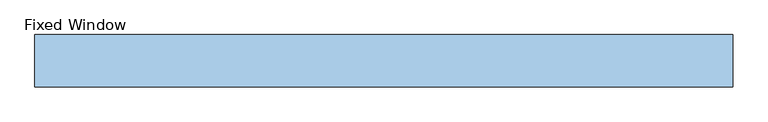
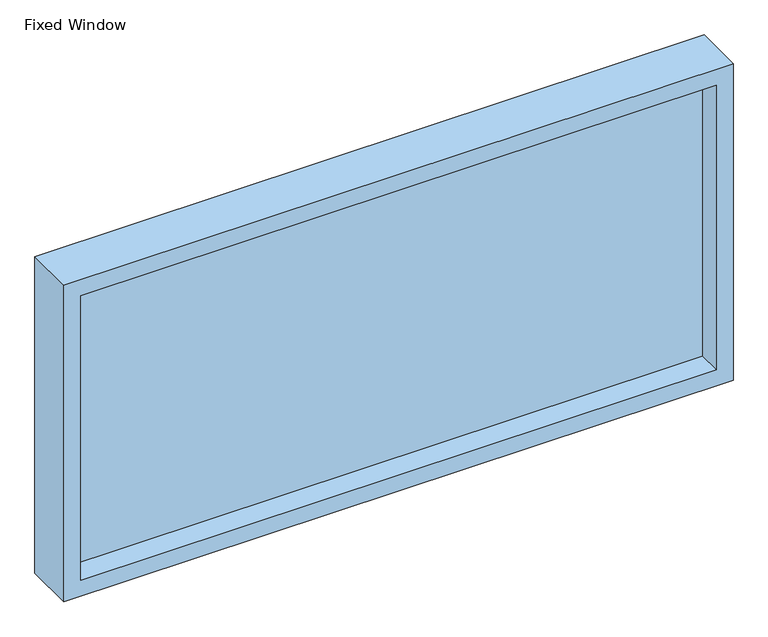
"""IFC4 building model written with IfcOpenShell, lengths in millimetres: window geometry, Fixed Window : H_WD_AR_B11_Fix_Steel Window_SG_W2000xH1000."""

import ifcopenshell
import ifcopenshell.guid

model = None  # the IFC model being written
_history = None  # IfcOwnerHistory: only IFC2X3 demands one
_inside = {}  # id of a spatial element -> (the spatial element, [elements in it])
_under = {}  # id of a project, library or spatial element -> (it, [spatial elements below it])
_declared = {}  # id of a project -> (the project, [libraries it declares])
_typed = {}  # id of a type object -> (the type object, [elements of that type])
_made_of = {}  # id of a material, layer set ... -> (it, [elements and type objects made of it])


def new_model(schema):
    """Start an empty IFC model of exactly this schema.

    Asked for "IFC4X3", IfcOpenShell would pick the latest addendum, in which some entities
    have other attributes; the version numbers below select the first issue.
    IFC2X3 requires an IfcOwnerHistory on every rooted entity: one is made here for all.
    """
    global model, _history
    if schema == "IFC4X3":
        model = ifcopenshell.file(schema_version=(4, 3, 0, 0))
    else:
        model = ifcopenshell.file(schema=schema)
    _inside.clear()
    _under.clear()
    _declared.clear()
    _typed.clear()
    _made_of.clear()
    _history = None
    if model.schema == "IFC2X3":
        org = make("IfcOrganization", Name="unknown")
        user = make(
            "IfcPersonAndOrganization",
            ThePerson=make("IfcPerson", FamilyName="unknown"),
            TheOrganization=org,
        )
        app = make(
            "IfcApplication",
            ApplicationDeveloper=org,
            Version="unknown",
            ApplicationFullName="unknown",
            ApplicationIdentifier="unknown",
        )
        _history = make(
            "IfcOwnerHistory",
            OwningUser=user,
            OwningApplication=app,
            ChangeAction="ADDED",
            CreationDate=0,
        )
    return model


def make(cls, **values):
    """One entity of the class cls with the attributes given. An attribute that is None is left unset."""
    return model.create_entity(
        cls, **{name: value for name, value in values.items() if value is not None}
    )


def rooted(cls, **values):
    """An entity with a GlobalId (a new one), such as an element, a storey or a relation."""
    return make(cls, GlobalId=ifcopenshell.guid.new(), OwnerHistory=_history, **values)


def si_unit(unit_type, name, prefix=None):
    """IfcSIUnit, for example si_unit("LENGTHUNIT", "METRE", prefix="MILLI")."""
    return make("IfcSIUnit", UnitType=unit_type, Prefix=prefix, Name=name)


def assignment(units):
    """IfcUnitAssignment: the units of a project."""
    return None if units is None else make("IfcUnitAssignment", Units=units)


def point(xyz):
    """IfcCartesianPoint."""
    return None if xyz is None else make("IfcCartesianPoint", Coordinates=xyz)


def direction(xyz):
    """IfcDirection."""
    return None if xyz is None else make("IfcDirection", DirectionRatios=xyz)


def frame(location, z_axis=None, x_axis=None):
    """IfcAxis2Placement3D, a coordinate frame: its origin and axes. An axis left out is left unset."""
    return make(
        "IfcAxis2Placement3D",
        Location=point(location),
        Axis=direction(z_axis),
        RefDirection=direction(x_axis),
    )


def origin():
    """The frame at (0, 0, 0) with its axes left unset."""
    return frame((0.0, 0.0, 0.0))


def place(relative_to, where):
    """IfcLocalPlacement: puts the frame where relative to a parent placement (None: the world)."""
    return make(
        "IfcLocalPlacement", PlacementRelTo=relative_to, RelativePlacement=where
    )


def context(
    kind, dimensions, precision=None, world=None, true_north=None, identifier=None
):
    """IfcGeometricRepresentationContext, for example the 3D "Model" context."""
    return make(
        "IfcGeometricRepresentationContext",
        ContextIdentifier=identifier,
        ContextType=kind,
        CoordinateSpaceDimension=dimensions,
        Precision=precision,
        WorldCoordinateSystem=world,
        TrueNorth=true_north,
    )


def project(units=None, contexts=None):
    """IfcProject with its units and contexts."""
    return rooted(
        "IfcProject",
        Name="project",
        RepresentationContexts=contexts,
        UnitsInContext=assignment(units),
    )


def spatial(cls, under=None, at=None, **own):
    """A site, building, storey or space (cls), placed at a placement, below another one or the project."""
    s = rooted(cls, ObjectPlacement=at, **own)
    if under is not None:
        _under.setdefault(under.id(), (under, []))[1].append(s)
    return s


def polyline(points):
    """IfcPolyline through the points."""
    return make("IfcPolyline", Points=[point(p) for p in points])


def outline(outer, holes=None, kind="AREA"):
    """IfcArbitraryClosedProfileDef: a profile drawn as a closed curve; with holes, ...WithVoids."""
    if holes is None:
        return make("IfcArbitraryClosedProfileDef", ProfileType=kind, OuterCurve=outer)
    return make(
        "IfcArbitraryProfileDefWithVoids",
        ProfileType=kind,
        OuterCurve=outer,
        InnerCurves=holes,
    )


def extrude(swept, where, along, depth):
    """IfcExtrudedAreaSolid: the profile swept, set in the frame where, extruded along a direction by depth."""
    return make(
        "IfcExtrudedAreaSolid",
        SweptArea=swept,
        Position=where,
        ExtrudedDirection=direction(along),
        Depth=depth,
    )


def shape(context_of_items, identifier, shape_type, items):
    """IfcShapeRepresentation: the items that make up one representation, for example the "Body"."""
    return make(
        "IfcShapeRepresentation",
        ContextOfItems=context_of_items,
        RepresentationIdentifier=identifier,
        RepresentationType=shape_type,
        Items=items,
    )


def source(mapping_origin, context_of_items, identifier, shape_type, items):
    """IfcRepresentationMap: a shape defined once, which mapped items show again and again."""
    return make(
        "IfcRepresentationMap",
        MappingOrigin=mapping_origin,
        MappedRepresentation=shape(context_of_items, identifier, shape_type, items),
    )


def transform(
    local_origin,
    x_axis=None,
    y_axis=None,
    z_axis=None,
    scale=None,
    scale2=None,
    scale3=None,
    uniform=True,
):
    """IfcCartesianTransformationOperator3D, or its non-uniform kind. x_axis, y_axis, z_axis: its Axis1, 2, 3."""
    if uniform:
        return make(
            "IfcCartesianTransformationOperator3D",
            Axis1=direction(x_axis),
            Axis2=direction(y_axis),
            LocalOrigin=point(local_origin),
            Scale=scale,
            Axis3=direction(z_axis),
        )
    return make(
        "IfcCartesianTransformationOperator3DnonUniform",
        Axis1=direction(x_axis),
        Axis2=direction(y_axis),
        LocalOrigin=point(local_origin),
        Scale=scale,
        Axis3=direction(z_axis),
        Scale2=scale2,
        Scale3=scale3,
    )


def mapped(mapping_source, mapping_target):
    """IfcMappedItem: shows the shape of a source again, moved by a transform."""
    return make(
        "IfcMappedItem", MappingSource=mapping_source, MappingTarget=mapping_target
    )


def made_of(thing, what):
    """Note that an element or type object is made of a material, layer set ...; save() writes the relation."""
    if what is not None:
        _made_of.setdefault(what.id(), (what, []))[1].append(thing)
    return thing


def element(
    cls,
    number,
    at=None,
    inside=None,
    cuts=None,
    type_object=None,
    material=None,
    context=None,
    identifier="Body",
    shape_type=None,
    held_by="IfcProductDefinitionShape",
    body=None,
    shapes=None,
    **own,
):
    """One element of the class cls, such as IfcWall. Its Tag is "e" and its number.

    at: its placement. inside: the storey or other place that contains it. cuts: it is an
    opening in that element (IfcRelVoidsElement). A single representation is given by context,
    identifier, shape_type and body (its items); several are given by shapes. held_by: the class
    of the entity that holds the representations. save() writes the other relations.
    """
    e = rooted(cls, Tag="e%d" % number, ObjectPlacement=at, **own)
    if body is not None:
        shapes = [shape(context, identifier, shape_type, body)]
    if shapes is not None:
        e.Representation = make(held_by, Representations=shapes)
    if inside is not None:
        _inside.setdefault(inside.id(), (inside, []))[1].append(e)
    if cuts is not None:
        rooted(
            "IfcRelVoidsElement", RelatingBuildingElement=cuts, RelatedOpeningElement=e
        )
    if type_object is not None:
        _typed.setdefault(type_object.id(), (type_object, []))[1].append(e)
    return made_of(e, material)


def aggregate(whole, parts):
    """IfcRelAggregates: a whole, such as a stair, and the parts it consists of."""
    return rooted("IfcRelAggregates", RelatingObject=whole, RelatedObjects=parts)


def save(model, path):
    """Write the relations noted so far, then the file.

    IfcRelAggregates (storeys below a building ...), IfcRelContainedInSpatialStructure (elements
    in a storey), IfcRelDefinesByType, IfcRelAssociatesMaterial and IfcRelDeclares: one each for
    every whole, place, type object, material and project.
    """
    for whole, parts in _under.values():
        aggregate(whole, parts)
    for where, things in _inside.values():
        rooted(
            "IfcRelContainedInSpatialStructure",
            RelatedElements=things,
            RelatingStructure=where,
        )
    for kind, things in _typed.values():
        rooted("IfcRelDefinesByType", RelatedObjects=things, RelatingType=kind)
    for what, things in _made_of.values():
        rooted("IfcRelAssociatesMaterial", RelatedObjects=things, RelatingMaterial=what)
    for by, libraries in _declared.values():
        rooted("IfcRelDeclares", RelatingContext=by, RelatedDefinitions=libraries)
    model.write(path)


def fixed_window_a76b3388(model_context):
    return source(origin(), model_context, "Body", "SweptSolid", [
        extrude(outline(polyline([(-950.0, 3.0), (950.0, 3.0), (950.0, -3.0), (-950.0, -3.0), (-950.0, 3.0)])), frame((0.0, 0.0, 850.0), z_axis=(0.0, 0.0, 1.0), x_axis=(1.0, 0.0, 0.0)), (0.0, 0.0, 1.0), 900.0),
        extrude(outline(polyline([(1800.0, -1000.0), (800.0, -1000.0), (800.0, 1000.0), (1800.0, 1000.0), (1800.0, -1000.0)]), holes=[polyline([(1750.0, -950.0), (1750.0, 950.0), (850.0, 950.0), (850.0, -950.0), (1750.0, -950.0)])]), frame((0.0, -75.0, 0.0), z_axis=(0.0, 1.0, 0.0), x_axis=(0.0, 0.0, 1.0)), (0.0, 0.0, 1.0), 150.0),
    ])


if __name__ == "__main__":
    model = new_model("IFC4")
    model_context = context("Model", 3, world=origin())
    ifc_project = project(units=[si_unit("LENGTHUNIT", "METRE", prefix="MILLI")], contexts=[model_context])
    site = spatial("IfcSite", under=ifc_project)
    building = spatial("IfcBuilding", under=site)
    placement = place(None, origin())
    fixed_window_shape = fixed_window_a76b3388(model_context)
    element("IfcWindow", 1, ObjectType="Fixed Window : H_WD_AR_B11_Fix_Steel Window_SG_W2000xH1000", at=placement, inside=building, context=model_context, shape_type="MappedRepresentation", body=[
        mapped(fixed_window_shape, transform((0.0, 0.0, 0.0), x_axis=(1.0, 0.0, 0.0), y_axis=(0.0, 1.0, 0.0), z_axis=(0.0, 0.0, 1.0))),
    ])
    save(model, "model.ifc")

# Revit data of these elements
# Type "Fixed Window : H_WD_AR_B11_Fix_Steel Window_SG_W2000xH1000"
#   Description = "PVC Frame + 2 x T=6mm + T12mm Air Space"
#   Type Mark = "AW"
#   Analytic Construction = "<None>"
#   창 두께 = 150 mm
#   Height = 1000 mm
#   절반 창 두께 = 75 mm
#   기본 씰 높이 = 800 mm
#   Width = 2000 mm
#   Define Thermal Properties by = 1
#   창 패널 = none
#   창 프레임 = none
#   Wall Closure = (empty or 0)
